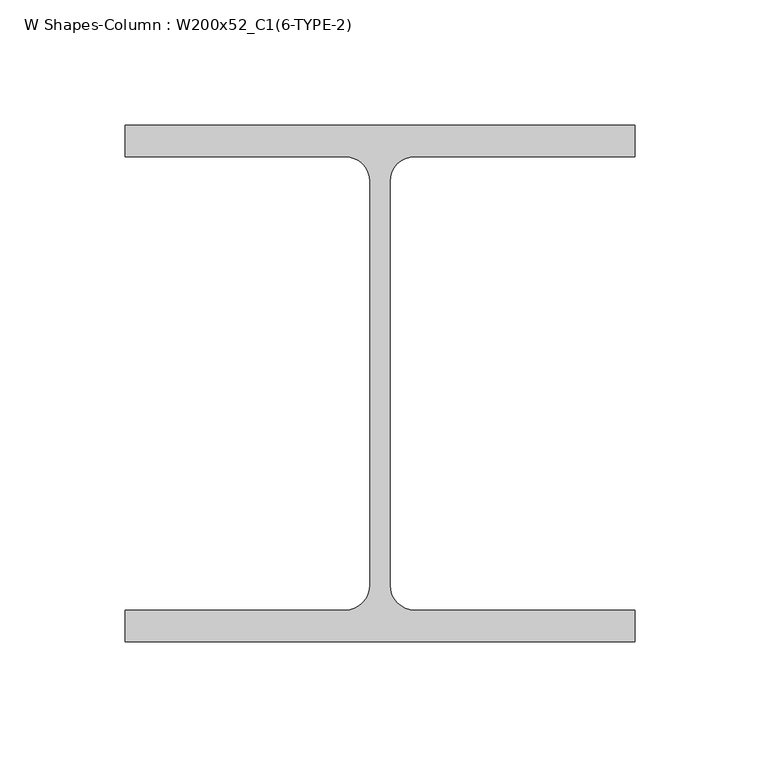
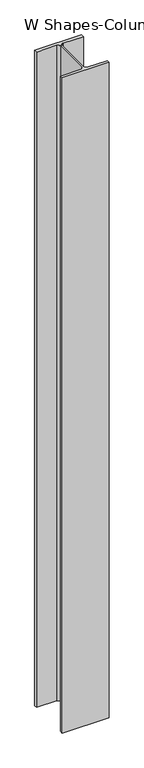
"""IFC4 building model written with IfcOpenShell, lengths in millimetres: column geometry, W Shapes-Column : W200x52_C1(6-TYPE-2)."""

from ifc_helpers import new_model, si_unit, point, frame, frame_2d, origin, place, context, project, spatial, polyline, circle_curve, trimmed, segment, composite_curve, outline, extrude, source, transform, mapped, element, save


def w_shapes_column_w200x52_c1_6_type_2_e34d810c(model_context):
    return source(origin(), model_context, "Body", "SweptSolid", [
        extrude(outline(composite_curve([segment(polyline([(101.854, -103.124), (-101.854, -103.124), (-101.854, -90.551), (-13.9446, -90.551)]), True, "CONTINUOUS"), segment(trimmed(circle_curve(frame_2d((-13.9446, -80.5434)), 10.0076), [point((-13.9446, -90.551))], [point((-3.937, -80.5434))], True, "CARTESIAN"), True, "CONTINUOUS"), segment(polyline([(-3.937, -80.5434), (-3.937, 80.5434)]), True, "CONTINUOUS"), segment(trimmed(circle_curve(frame_2d((-13.9446, 80.5434)), 10.0076), [point((-3.937, 80.5434))], [point((-13.9446, 90.551))], True, "CARTESIAN"), True, "CONTINUOUS"), segment(polyline([(-13.9446, 90.551), (-101.854, 90.551), (-101.854, 103.124), (101.854, 103.124), (101.854, 90.551), (13.9446, 90.551)]), True, "CONTINUOUS"), segment(trimmed(circle_curve(frame_2d((13.9446, 80.5434)), 10.0076), [point((13.9446, 90.551))], [point((3.937, 80.5434))], True, "CARTESIAN"), True, "CONTINUOUS"), segment(polyline([(3.937, 80.5434), (3.937, -80.5434)]), True, "CONTINUOUS"), segment(trimmed(circle_curve(frame_2d((13.9446, -80.5434)), 10.0076), [point((3.937, -80.5434))], [point((13.9446, -90.551))], True, "CARTESIAN"), True, "CONTINUOUS"), segment(polyline([(13.9446, -90.551), (101.854, -90.551), (101.854, -103.124)]), True, "CONTINUOUS")], self_intersect=False)), frame((0.0, 0.0, 6240.0), z_axis=(0.0, 0.0, 1.0), x_axis=(1.0, 0.0, 0.0)), (0.0, 0.0, 1.0), 3000.0),
    ])


if __name__ == "__main__":
    model = new_model("IFC4")
    model_context = context("Model", 3, world=origin())
    ifc_project = project(units=[si_unit("LENGTHUNIT", "METRE", prefix="MILLI")], contexts=[model_context])
    site = spatial("IfcSite", under=ifc_project)
    building = spatial("IfcBuilding", under=site)
    placement = place(None, origin())
    w_shapes_column_w200x52_c1_6_type_2_shape = w_shapes_column_w200x52_c1_6_type_2_e34d810c(model_context)
    element("IfcColumn", 1, ObjectType="W Shapes-Column : W200x52_C1(6-TYPE-2)", at=placement, inside=building, context=model_context, shape_type="MappedRepresentation", body=[
        mapped(w_shapes_column_w200x52_c1_6_type_2_shape, transform((0.0, 0.0, 0.0), x_axis=(1.0, 0.0, 0.0), y_axis=(0.0, 1.0, 0.0), z_axis=(0.0, 0.0, 1.0))),
    ])
    save(model, "model.ifc")

# Revit data of these elements
# Type "W Shapes-Column : W200x52_C1(6-TYPE-2)"
#   Section Name Key = "W8X35"
#   Assembly Code = "B10"
#   Width = 20.3708 cm
#   Web Thickness = 0.7874 cm
#   Web Fillet = 1.0008 cm
#   Warping Constant = 166223.7 cm⁶
#   Torsional Moment of Inertia = 32.0082 cm⁴
#   Section Area = 66.4515 cm²
#   Plastic Modulus weak axis = 263.832 cm³
#   Plastic Modulus strong axis = 568.631 cm³
#   Perimeter = 1.1936 m²/m
#   Nominal Weight = 52.0857 kgf/m
#   Moment of Inertia weak axis = 1773.15 cm⁴
#   Moment of Inertia strong axis = 5286.14 cm⁴
#   Height = 20.6248 cm
#   Flange Thickness = 1.2573 cm
#   Elastic Modulus weak axis = 173.703 cm³
#   Elastic Modulus strong axis = 511.276 cm³
#   Clear Web Height = 14.605 cm
#   Centroid Vertical = 10.3124 cm
#   Centroid Horizontal = 10.1854 cm
#   Bolt Spacing = 13.97 cm
#   Structural Material [instance default] = Steel ASTM A992
#   Principal Axes Angle = 0
# Element 1 (IfcColumn, "W Shapes-Column : W200x52_C1(6-TYPE-2)")
#   Structural Material = none
# Materials
#   "Steel ASTM A992": class "Metal", colour RGB 199 199 199, transparency 0, Description = "Structural steel 50ksi", Cost = 0
